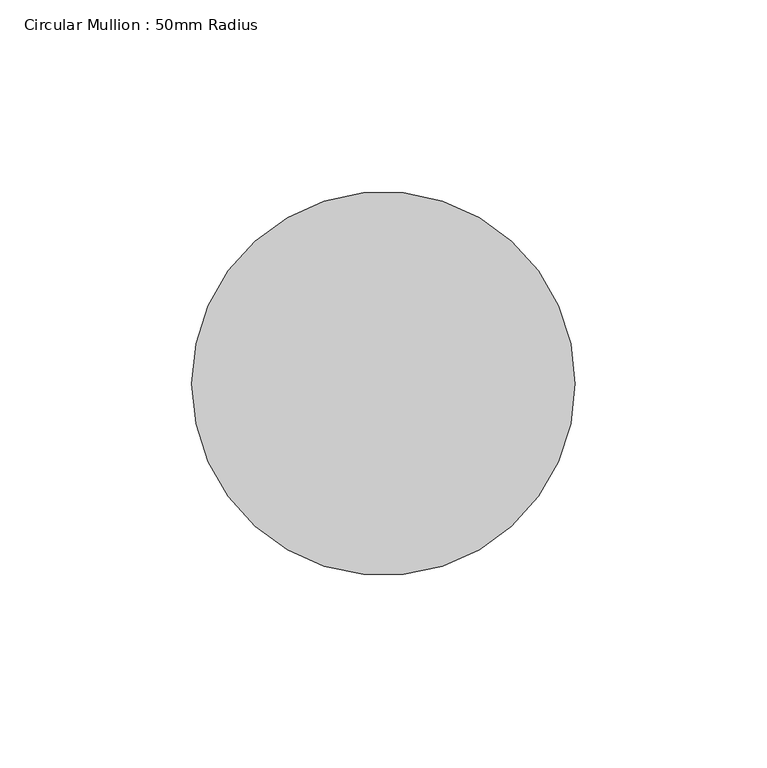
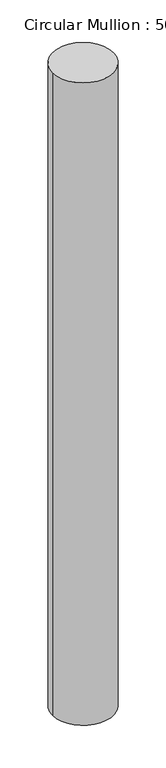
"""IFC4 building model written with IfcOpenShell, lengths in millimetres: member geometry, Circular Mullion : 50mm Radius."""

from ifc_helpers import new_model, si_unit, point, frame, origin, origin_2d, place, context, project, spatial, circle_curve, trimmed, segment, composite_curve, outline, extrude, source, transform, mapped, element, save


def circular_mullion_50mm_radius_76b0b386(model_context):
    return source(origin(), model_context, "Body", "SweptSolid", [
        extrude(outline(composite_curve([segment(trimmed(circle_curve(origin_2d(), 50.0), [point((50.0, 0.0))], [point((-50.0, 0.0))], False, "CARTESIAN"), True, "CONTINUOUS"), segment(trimmed(circle_curve(origin_2d(), 50.0), [point((-50.0, 0.0))], [point((50.0, 0.0))], False, "CARTESIAN"), True, "CONTINUOUS")], self_intersect=False)), frame((0.0, 0.0, -1115.1652049), z_axis=(0.0, 0.0, 1.0), x_axis=(1.0, 0.0, 0.0)), (0.0, 0.0, 1.0), 1115.1652049),
    ])


if __name__ == "__main__":
    model = new_model("IFC4")
    model_context = context("Model", 3, world=origin())
    ifc_project = project(units=[si_unit("LENGTHUNIT", "METRE", prefix="MILLI")], contexts=[model_context])
    site = spatial("IfcSite", under=ifc_project)
    building = spatial("IfcBuilding", under=site)
    placement = place(None, origin())
    circular_mullion_50mm_radius_shape = circular_mullion_50mm_radius_76b0b386(model_context)
    element("IfcMember", 1, ObjectType="Circular Mullion : 50mm Radius", at=placement, inside=building, context=model_context, shape_type="MappedRepresentation", body=[
        mapped(circular_mullion_50mm_radius_shape, transform((0.0, 0.0, 0.0), x_axis=(1.0, 0.0, 0.0), y_axis=(0.0, 1.0, 0.0), z_axis=(0.0, 0.0, 1.0))),
    ])
    save(model, "model.ifc")

# Revit data of these elements
# Type "Circular Mullion : 50mm Radius"
#   built-in parameter 1007350 = 0.164042 (stored number, unit not read)
# Element 1 (IfcMember, "Circular Mullion : 50mm Radius")
#   Materials on its faces: "Aluminium"
# Materials
#   "Aluminium": class "Metal", colour RGB 247 247 247, transparency 0, Description = "Aluminium 6061", Cost = 0
